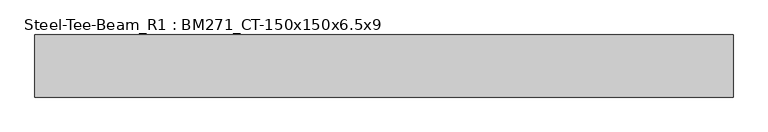
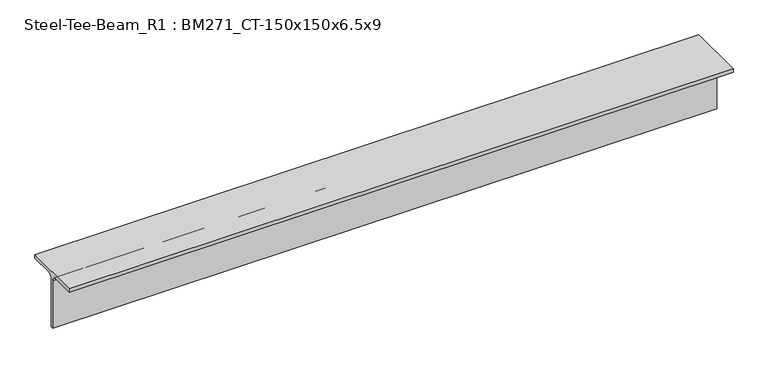
"""IFC4 building model written with IfcOpenShell, lengths in millimetres: member geometry, Steel-Tee-Beam_R1 : BM271_CT-150x150x6.5x9."""

from ifc_helpers import new_model, si_unit, point, frame, frame_2d, origin, place, context, project, spatial, polyline, circle_curve, trimmed, segment, composite_curve, outline, extrude, source, transform, mapped, element, save


def steel_tee_beam_r1_bm271_ct_150x150x6_5x9_4fef89d3(model_context):
    return source(origin(), model_context, "Body", "SweptSolid", [
        extrude(outline(composite_curve([segment(polyline([(-75.0, 75.0), (75.0, 75.0), (75.0, 66.0), (16.25, 66.0)]), True, "CONTINUOUS"), segment(trimmed(circle_curve(frame_2d((16.25, 53.0)), 13.0), [point((16.25, 66.0))], [point((3.25, 53.0))], True, "CARTESIAN"), True, "CONTINUOUS"), segment(polyline([(3.25, 53.0), (3.25, -75.0), (-3.25, -75.0), (-3.25, 53.0)]), True, "CONTINUOUS"), segment(trimmed(circle_curve(frame_2d((-16.25, 53.0)), 13.0), [point((-3.25, 53.0))], [point((-16.25, 66.0))], True, "CARTESIAN"), True, "CONTINUOUS"), segment(polyline([(-16.25, 66.0), (-75.0, 66.0), (-75.0, 75.0)]), True, "CONTINUOUS")], self_intersect=False)), frame((-842.322898, 0.0, 0.0), z_axis=(1.0, 0.0, 0.0), x_axis=(0.0, 1.0, 0.0)), (0.0, 0.0, 1.0), 1684.6457959),
    ])


if __name__ == "__main__":
    model = new_model("IFC4")
    model_context = context("Model", 3, world=origin())
    ifc_project = project(units=[si_unit("LENGTHUNIT", "METRE", prefix="MILLI")], contexts=[model_context])
    site = spatial("IfcSite", under=ifc_project)
    building = spatial("IfcBuilding", under=site)
    placement = place(None, origin())
    steel_tee_beam_r1_bm271_ct_150x150x6_5x9_shape = steel_tee_beam_r1_bm271_ct_150x150x6_5x9_4fef89d3(model_context)
    element("IfcMember", 1, ObjectType="Steel-Tee-Beam_R1 : BM271_CT-150x150x6.5x9", at=placement, inside=building, context=model_context, shape_type="MappedRepresentation", body=[
        mapped(steel_tee_beam_r1_bm271_ct_150x150x6_5x9_shape, transform((0.0, 0.0, 0.0), x_axis=(1.0, 0.0, 0.0), y_axis=(0.0, 1.0, 0.0), z_axis=(0.0, 0.0, 1.0))),
    ])
    save(model, "model.ifc")

# Revit data of these elements
# Type "Steel-Tee-Beam_R1 : BM271_CT-150x150x6.5x9"
#   Keynote = "CT-150x150x6.5x9"
#   Surface Area = 0.588841 m²/m
#   Section Area = 23.3904 cm²
#   Mass per Unit Length = 18.3614 kg/m
#   Length [instance default] = 1.5240 m
#   bf = 0.1500 m
#   d = 0.1500 m
#   k = 0.0220 m
#   r = 0.0130 m
#   tf = 0.0090 m
#   tw = 0.0065 m
#   hec_material4 [instance default] = none
#   hec_material3 [instance default] = none
#   hec_material2 [instance default] = none
#   hec_material1 [instance default] = none
#   Structural Material [instance default] = Steel, 45-345
#   Assembly Code = ""
# Element 1 (IfcMember, "Steel-Tee-Beam_R1 : BM271_CT-150x150x6.5x9")
#   Structural Material = none
# Materials
#   "Steel, 45-345": class "Metal", colour RGB 189 187 185, transparency 0, Description = "Steel 345 MPa", Cost = 0
